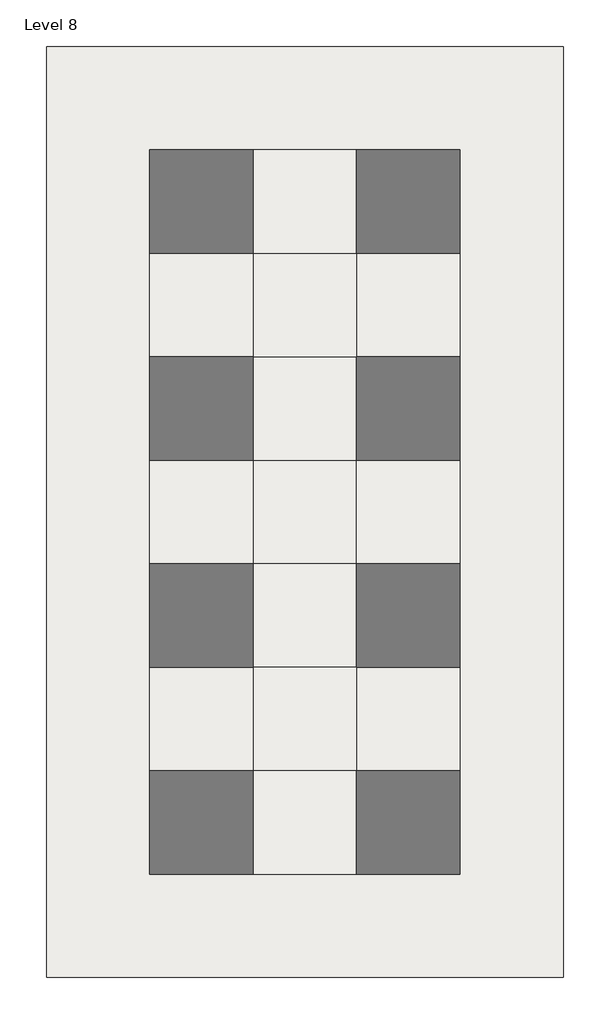
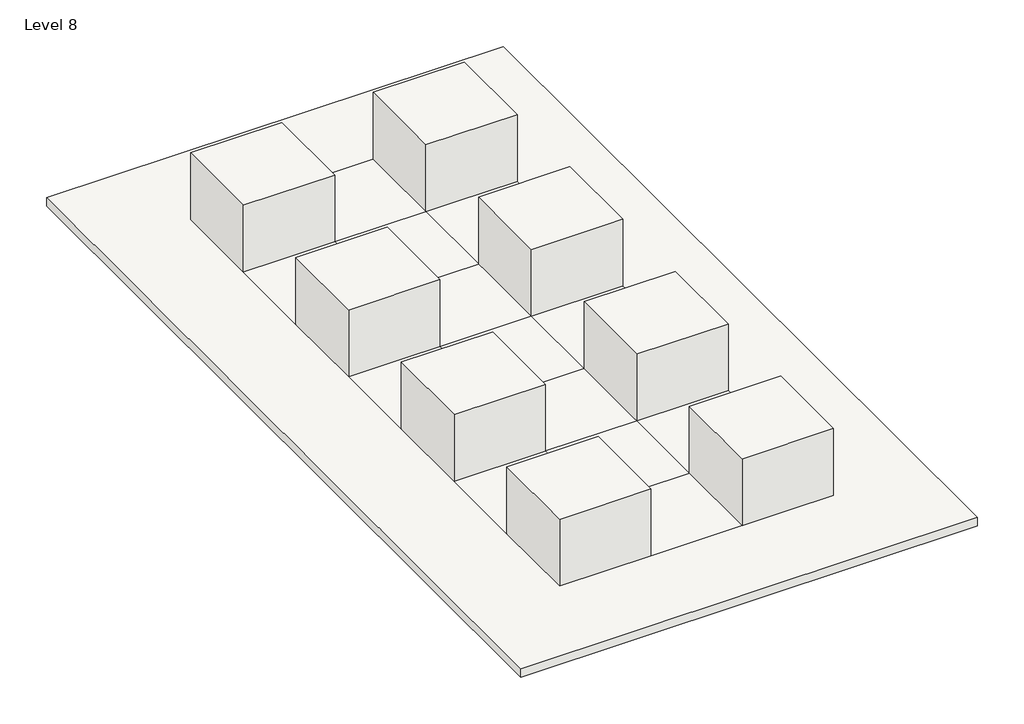
# One storey: 9 roofs.
"""IFC4 building model written with IfcOpenShell, lengths in millimetres."""

from ifc_helpers import new_model, si_unit, origin, place, context, project, spatial, faceted_brep, element, save

model = new_model("IFC4")

# Units and contexts
model_context = context("Model", 3, world=origin())
ifc_project = project(units=[si_unit("LENGTHUNIT", "METRE", prefix="MILLI")], contexts=[model_context])

# Site, building, storey
site = spatial("IfcSite", under=ifc_project)
building = spatial("IfcBuilding", under=site)
storey = spatial("IfcBuildingStorey", under=building, Name="Level 8", Elevation=32000.0)

# Roofs
placement = place(None, origin())
element("IfcRoof", 1, ObjectType="Bauder_RoofCoveringSystem_IntensiveGreenRoofSystem", at=placement, inside=storey, context=model_context, shape_type="Brep", body=[
    faceted_brep([(-674.7340554, 1676.2074539, 32000.0), (1325.2659446, 1676.2074539, 32000.0), (1325.2659446, -323.7925461, 32000.0), (-674.7340554, -323.7925461, 32000.0), (1325.2659446, 1676.2074539, 33749.8), (-674.7340554, 1676.2074539, 33749.8), (-674.7340554, -323.7925461, 33749.8), (1325.2659446, -323.7925461, 33749.8), (1325.2659446, 1676.2074539, 32200.0), (-674.7340554, 1676.2074539, 32200.0), (-674.7340554, -323.7925461, 32200.0), (1325.2659446, -323.7925461, 32200.0)], [[[0, 1, 2, 3]], [[4, 5, 6, 7]], [[5, 4, 8, 1, 0, 9]], [[6, 5, 9, 0, 3, 10]], [[7, 6, 10, 3, 2, 11]], [[4, 7, 11, 2, 1, 8]]]),
])
element("IfcRoof", 2, ObjectType="Bauder_RoofCoveringSystem_IntensiveGreenRoofSystem", at=placement, inside=storey, context=model_context, shape_type="Brep", body=[
    faceted_brep([(3325.2659446, 1676.2074539, 32000.0), (5325.2659446, 1676.2074539, 32000.0), (5325.2659446, -323.7925461, 32000.0), (3325.2659446, -323.7925461, 32000.0), (5325.2659446, 1676.2074539, 33749.8), (3325.2659446, 1676.2074539, 33749.8), (3325.2659446, -323.7925461, 33749.8), (5325.2659446, -323.7925461, 33749.8), (5325.2659446, 1676.2074539, 32200.0), (3325.2659446, 1676.2074539, 32200.0), (3325.2659446, -323.7925461, 32200.0), (5325.2659446, -323.7925461, 32200.0)], [[[0, 1, 2, 3]], [[4, 5, 6, 7]], [[5, 4, 8, 1, 0, 9]], [[6, 5, 9, 0, 3, 10]], [[7, 6, 10, 3, 2, 11]], [[4, 7, 11, 2, 1, 8]]]),
])
element("IfcRoof", 3, ObjectType="Bauder_RoofCoveringSystem_IntensiveGreenRoofSystem", at=placement, inside=storey, context=model_context, shape_type="Brep", body=[
    faceted_brep([(3325.2659446, -2323.7925461, 32000.0), (5325.2659446, -2323.7925461, 32000.0), (5325.2659446, -4323.7925461, 32000.0), (3325.2659446, -4323.7925461, 32000.0), (5325.2659446, -2323.7925461, 33749.8), (3325.2659446, -2323.7925461, 33749.8), (3325.2659446, -4323.7925461, 33749.8), (5325.2659446, -4323.7925461, 33749.8), (5325.2659446, -2323.7925461, 32200.0), (3325.2659446, -2323.7925461, 32200.0), (3325.2659446, -4323.7925461, 32200.0), (5325.2659446, -4323.7925461, 32200.0)], [[[0, 1, 2, 3]], [[4, 5, 6, 7]], [[5, 4, 8, 1, 0, 9]], [[6, 5, 9, 0, 3, 10]], [[7, 6, 10, 3, 2, 11]], [[4, 7, 11, 2, 1, 8]]]),
])
element("IfcRoof", 4, ObjectType="Bauder_RoofCoveringSystem_IntensiveGreenRoofSystem", at=placement, inside=storey, context=model_context, shape_type="Brep", body=[
    faceted_brep([(3325.2659446, -6323.7925461, 32000.0), (5325.2659446, -6323.7925461, 32000.0), (5325.2659446, -8323.7925461, 32000.0), (3325.2659446, -8323.7925461, 32000.0), (5325.2659446, -6323.7925461, 33749.8), (3325.2659446, -6323.7925461, 33749.8), (3325.2659446, -8323.7925461, 33749.8), (5325.2659446, -8323.7925461, 33749.8), (5325.2659446, -6323.7925461, 32200.0), (3325.2659446, -6323.7925461, 32200.0), (3325.2659446, -8323.7925461, 32200.0), (5325.2659446, -8323.7925461, 32200.0)], [[[0, 1, 2, 3]], [[4, 5, 6, 7]], [[5, 4, 8, 1, 0, 9]], [[6, 5, 9, 0, 3, 10]], [[7, 6, 10, 3, 2, 11]], [[4, 7, 11, 2, 1, 8]]]),
])
element("IfcRoof", 5, ObjectType="Bauder_RoofCoveringSystem_IntensiveGreenRoofSystem", at=placement, inside=storey, context=model_context, shape_type="Brep", body=[
    faceted_brep([(3325.2659446, -10323.7925461, 32000.0), (5325.2659446, -10323.7925461, 32000.0), (5325.2659446, -12323.7925461, 32000.0), (3325.2659446, -12323.7925461, 32000.0), (5325.2659446, -10323.7925461, 33749.8), (3325.2659446, -10323.7925461, 33749.8), (3325.2659446, -12323.7925461, 33749.8), (5325.2659446, -12323.7925461, 33749.8), (5325.2659446, -10323.7925461, 32200.0), (3325.2659446, -10323.7925461, 32200.0), (3325.2659446, -12323.7925461, 32200.0), (5325.2659446, -12323.7925461, 32200.0)], [[[0, 1, 2, 3]], [[4, 5, 6, 7]], [[5, 4, 8, 1, 0, 9]], [[6, 5, 9, 0, 3, 10]], [[7, 6, 10, 3, 2, 11]], [[4, 7, 11, 2, 1, 8]]]),
])
element("IfcRoof", 6, ObjectType="Bauder_RoofCoveringSystem_IntensiveGreenRoofSystem", at=placement, inside=storey, context=model_context, shape_type="Brep", body=[
    faceted_brep([(-674.7340554, -10323.7925461, 32000.0), (1325.2659446, -10323.7925461, 32000.0), (1325.2659446, -12323.7925461, 32000.0), (-674.7340554, -12323.7925461, 32000.0), (1325.2659446, -10323.7925461, 33749.8), (-674.7340554, -10323.7925461, 33749.8), (-674.7340554, -12323.7925461, 33749.8), (1325.2659446, -12323.7925461, 33749.8), (1325.2659446, -10323.7925461, 32200.0), (-674.7340554, -10323.7925461, 32200.0), (-674.7340554, -12323.7925461, 32200.0), (1325.2659446, -12323.7925461, 32200.0)], [[[0, 1, 2, 3]], [[4, 5, 6, 7]], [[5, 4, 8, 1, 0, 9]], [[6, 5, 9, 0, 3, 10]], [[7, 6, 10, 3, 2, 11]], [[4, 7, 11, 2, 1, 8]]]),
])
element("IfcRoof", 7, ObjectType="Bauder_RoofCoveringSystem_IntensiveGreenRoofSystem", at=placement, inside=storey, context=model_context, shape_type="Brep", body=[
    faceted_brep([(-674.7340554, -6323.7925461, 32000.0), (1325.2659446, -6323.7925461, 32000.0), (1325.2659446, -8323.7925461, 32000.0), (-674.7340554, -8323.7925461, 32000.0), (1325.2659446, -6323.7925461, 33749.8), (-674.7340554, -6323.7925461, 33749.8), (-674.7340554, -8323.7925461, 33749.8), (1325.2659446, -8323.7925461, 33749.8), (1325.2659446, -6323.7925461, 32200.0), (-674.7340554, -6323.7925461, 32200.0), (-674.7340554, -8323.7925461, 32200.0), (1325.2659446, -8323.7925461, 32200.0)], [[[0, 1, 2, 3]], [[4, 5, 6, 7]], [[5, 4, 8, 1, 0, 9]], [[6, 5, 9, 0, 3, 10]], [[7, 6, 10, 3, 2, 11]], [[4, 7, 11, 2, 1, 8]]]),
])
element("IfcRoof", 8, ObjectType="Bauder_RoofCoveringSystem_IntensiveGreenRoofSystem", at=placement, inside=storey, context=model_context, shape_type="Brep", body=[
    faceted_brep([(-674.7340554, -2323.7925461, 32000.0), (1325.2659446, -2323.7925461, 32000.0), (1325.2659446, -4323.7925461, 32000.0), (-674.7340554, -4323.7925461, 32000.0), (1325.2659446, -2323.7925461, 33749.8), (-674.7340554, -2323.7925461, 33749.8), (-674.7340554, -4323.7925461, 33749.8), (1325.2659446, -4323.7925461, 33749.8), (1325.2659446, -2323.7925461, 32200.0), (-674.7340554, -2323.7925461, 32200.0), (-674.7340554, -4323.7925461, 32200.0), (1325.2659446, -4323.7925461, 32200.0)], [[[0, 1, 2, 3]], [[4, 5, 6, 7]], [[5, 4, 8, 1, 0, 9]], [[6, 5, 9, 0, 3, 10]], [[7, 6, 10, 3, 2, 11]], [[4, 7, 11, 2, 1, 8]]]),
])
element("IfcRoof", 9, ObjectType="Roof_Concrete-200mm", at=placement, inside=storey, context=model_context, shape_type="Brep", body=[
    faceted_brep([(-2674.7340554, -14323.7925461, 32200.0), (-2674.7340554, -14323.7925461, 32000.0), (7325.2659446, -14323.7925461, 32000.0), (7325.2659446, -14323.7925461, 32200.0), (-2674.7340554, 3676.2074539, 32200.0), (-2674.7340554, 3676.2074539, 32000.0), (7325.2659446, 3676.2074539, 32200.0), (7325.2659446, 3676.2074539, 32000.0), (3325.2659446, 1676.2074539, 32200.0), (1325.2659446, 1676.2074539, 32200.0), (1325.2659446, -323.7925461, 32200.0), (3325.2659446, -323.7925461, 32200.0), (1325.2659446, 1676.2074539, 32000.0), (3325.2659446, 1676.2074539, 32000.0), (3325.2659446, -323.7925461, 32000.0), (1325.2659446, -323.7925461, 32000.0), (1325.2659446, -2323.7925461, 32200.0), (-674.7340554, -323.7925461, 32200.0), (-674.7340554, -2323.7925461, 32200.0), (3325.2659446, -2323.7925461, 32200.0), (5325.2659446, -2323.7925461, 32200.0), (5325.2659446, -323.7925461, 32200.0), (-674.7340554, -2323.7925461, 32000.0), (-674.7340554, -323.7925461, 32000.0), (1325.2659446, -2323.7925461, 32000.0), (3325.2659446, -2323.7925461, 32000.0), (5325.2659446, -323.7925461, 32000.0), (5325.2659446, -2323.7925461, 32000.0), (1325.2659446, -4323.7925461, 32200.0), (3325.2659446, -4323.7925461, 32200.0), (3325.2659446, -4323.7925461, 32000.0), (1325.2659446, -4323.7925461, 32000.0), (1325.2659446, -6323.7925461, 32200.0), (-674.7340554, -4323.7925461, 32200.0), (-674.7340554, -6323.7925461, 32200.0), (5325.2659446, -6323.7925461, 32200.0), (5325.2659446, -4323.7925461, 32200.0), (3325.2659446, -6323.7925461, 32200.0), (-674.7340554, -6323.7925461, 32000.0), (-674.7340554, -4323.7925461, 32000.0), (1325.2659446, -6323.7925461, 32000.0), (3325.2659446, -6323.7925461, 32000.0), (5325.2659446, -4323.7925461, 32000.0), (5325.2659446, -6323.7925461, 32000.0), (1325.2659446, -12323.7925461, 32200.0), (3325.2659446, -12323.7925461, 32200.0), (3325.2659446, -10323.7925461, 32200.0), (1325.2659446, -10323.7925461, 32200.0), (3325.2659446, -12323.7925461, 32000.0), (1325.2659446, -12323.7925461, 32000.0), (1325.2659446, -10323.7925461, 32000.0), (3325.2659446, -10323.7925461, 32000.0), (1325.2659446, -8323.7925461, 32200.0), (-674.7340554, -8323.7925461, 32200.0), (-674.7340554, -10323.7925461, 32200.0), (3325.2659446, -8323.7925461, 32200.0), (5325.2659446, -10323.7925461, 32200.0), (5325.2659446, -8323.7925461, 32200.0), (-674.7340554, -10323.7925461, 32000.0), (-674.7340554, -8323.7925461, 32000.0), (1325.2659446, -8323.7925461, 32000.0), (3325.2659446, -8323.7925461, 32000.0), (5325.2659446, -8323.7925461, 32000.0), (5325.2659446, -10323.7925461, 32000.0), (-674.7340554, 1676.2074539, 32000.0), (-674.7340554, 1676.2074539, 32200.0), (5325.2659446, 1676.2074539, 32200.0), (5325.2659446, 1676.2074539, 32000.0), (5325.2659446, -12323.7925461, 32000.0), (5325.2659446, -12323.7925461, 32200.0), (-674.7340554, -12323.7925461, 32000.0), (-674.7340554, -12323.7925461, 32200.0)], [[[0, 1, 2, 3]], [[1, 0, 4, 5]], [[6, 7, 5, 4]], [[3, 2, 7, 6]], [[8, 9, 10, 11]], [[12, 13, 14, 15]], [[16, 10, 17, 18]], [[11, 10, 16, 19]], [[20, 21, 11, 19]], [[22, 23, 15, 24]], [[15, 14, 25, 24]], [[25, 14, 26, 27]], [[19, 16, 28, 29]], [[24, 25, 30, 31]], [[32, 28, 33, 34]], [[35, 36, 29, 37]], [[38, 39, 31, 40]], [[41, 30, 42, 43]], [[44, 45, 46, 47]], [[48, 49, 50, 51]], [[47, 52, 53, 54]], [[47, 46, 55, 52]], [[56, 57, 55, 46]], [[58, 59, 60, 50]], [[51, 50, 60, 61]], [[51, 61, 62, 63]], [[52, 55, 37, 32]], [[29, 28, 32, 37]], [[61, 60, 40, 41]], [[31, 30, 41, 40]], [[9, 12, 15, 10]], [[10, 15, 23, 17]], [[17, 23, 64, 65]], [[12, 9, 65, 64]], [[66, 67, 26, 21]], [[21, 26, 14, 11]], [[11, 14, 13, 8]], [[67, 66, 8, 13]], [[20, 27, 42, 36]], [[36, 42, 30, 29]], [[29, 30, 25, 19]], [[27, 20, 19, 25]], [[16, 24, 31, 28]], [[28, 31, 39, 33]], [[33, 39, 22, 18]], [[24, 16, 18, 22]], [[32, 40, 60, 52]], [[52, 60, 59, 53]], [[53, 59, 38, 34]], [[40, 32, 34, 38]], [[35, 43, 62, 57]], [[57, 62, 61, 55]], [[55, 61, 41, 37]], [[43, 35, 37, 41]], [[56, 63, 68, 69]], [[69, 68, 48, 45]], [[45, 48, 51, 46]], [[63, 56, 46, 51]], [[47, 50, 49, 44]], [[44, 49, 70, 71]], [[71, 70, 58, 54]], [[50, 47, 54, 58]], [[4, 0, 3, 6], [9, 8, 66, 21, 20, 36, 35, 57, 56, 69, 45, 44, 71, 54, 53, 34, 33, 18, 17, 65]], [[7, 2, 1, 5], [13, 12, 64, 23, 22, 39, 38, 59, 58, 70, 49, 48, 68, 63, 62, 43, 42, 27, 26, 67]]]),
])

save(model, "model.ifc")

# Revit data of these elements
# Type "Bauder_RoofCoveringSystem_IntensiveGreenRoofSystem"
#   Keynote = "Q37"
#   Type IFC Predefined Type = "FLAT_ROOF"
#   Export Type to IFC As = "IfcRoofType"
#   Model = "Bauder Intensive Landscaping and Substrate - Intensive Green Roof System"
#   Manufacturer = "Bauder Ltd"
#   Type Comments = "Intensive Green Roof System"
#   URL = "http://www.bauder.co.uk/"
#   Description = "Bauder Intensive GreenRoof system incorporating Intensive Landscaping with Intensive Substrate, Filter Fleece, Mineral Drain, DSE60 Polyethylene Drainage and Protection Layer, FSM 1100 protection mat and PE Foil Polyethylene Separation-Slip Layer"
#   Assembly Code = "B3010"
#   NBSDescription = "Intensive green roof system"
#   NBSReference = "45-40-47/110"
#   BIMObjectName = "Bauder_RoofCoveringSystem_IntensiveGreenRoofSystem"
#   AccessibilityPerformance = "n/a"
#   CodePerformance = "n/a"
#   Color = "n/a"
#   Constituents = "n/a"
#   DurationUnit = "Year"
#   ExpectedLife = "n/a"
#   Features = "This BIM Object must be supported by a project specific specification from Bauder, incorporating system build-up, detail design and performance calculations if a full Bauder system guarantee is required. Please contact your local Bauder Representative or technical@bauder.co.uk"
#   Finish = "n/a"
#   Grade = "n/a"
#   Material = "n/a"
#   ModelReference = "Bauder Intensive Landscaping and Substrate - Intensive Green Roof System"
#   Name = "RoofCoveringSystem_Bauder_IntensiveGreenRoofSystem"
#   ReplacementCost = "n/a"
#   Shape = "n/a"
#   Size = "n/a"
#   SustainabilityPerformance = "Bauder Germany ISO14001: Certificate No.: 70499/03-15 e, Bauder UK ISO14001:Certificate No. 19ACM6595R, EN1271, BREEAM Credits Available"
#   WarrantyDescription = "Guarantee options could include ‘Product’, ‘Product and Workmanship’ and ‘Product, Workmanship and Design’ Guarantees. All guarantees available for this system are subject to the works being carried out in accordance with the Bauder specification and being installed by a Bauder Approved installer. For full details and further information regarding guarantees and alternative systems please contact your local Bauder Representative or technical@bauder.co.uk"
#   WarrantyDurationLabor = "n/a"
#   WarrantyDurationParts = "n/a\r\nn/a"
#   WarrantyDurationUnit = "Year"
#   WarrantyGuarantorLabor = "n/a"
#   WarrantyGuarantorParts = "technical@bauder.co.uk"
#   Certification = "n/a"
#   EdgeRestraints = "Perforated edge trim where required, refer to Bauder Project Specific Specification"
#   MoistureControlDrainageAncillaries = "n/a"
#   MoistureControlDrainageLayer = "Bauder DSE60 60 mm Polyethylene Drainage and Protection Layer with Bauder Mineral Drain Single size stone aggregate infill"
#   MoistureControlFilterMembrane = "Bauder Filter Fleece 1 mm Polypropylene Filter Fleece"
#   MoistureControlMoistureRetentionMat = "n/a"
#   PlantingSystemsAntierosionMat = "Jute Net where exposed, refer to Bauder Project Specific Specification"
#   PlantingSystemsPlantingMedium = "Bauder Intensive Substrate Recycled crushed brick, expanded clay shale and composted pine bark"
#   PlantingSystemsVegetation = "Bauder Intensive Landscaping"
#   PlantingSystemsVegetationBarrier = "20-40 mm Rounded-Washed Stones, refer to Bauder Project Specific Specification"
#   ProjectSpecificationAndDesign = "This BIM Object must be supported by a project specific specification from Bauder, incorporating system build-up, detail design and performance calculations if a full Bauder system warranty is required. Please contact your local Bauder Representative or technical@bauder.co.uk"
#   ProtectionProtectionLayer = "BauderGREEN FSM 1100 Protection Mat"
#   ProtectionRootBarrier = "As per project specific Bauder Specification"
#   ProtectionSeparationLayer = "2 layers of Bauder PE Foil 0.2 mm Polyethylene Separation-Slip Layer"
#   SystemManufacturer = "Bauder Ltd"
#   WarrantyConsiderations = "All guarantees available for this system are subject to the works being carried out in accordance with the Bauder specification and being installed by a Bauder Approved installer. For full details and further information regarding guarantees and alternative systems please contact your local Bauder Representative or technical@bauder.co.uk"
#   Update = "1900-12-31T23:59:59"
#   Documentation = "https://www.bauder.co.uk/technical-centre/technical-literature/system-brochures"
#   DocumentReference = "http://www.bauder.co.uk/"
#   IfcExportAs = "IfcRoofType"
#   IfcExportType = "FLAT_ROOF"
#   MethodOfMesurement = "n/a"
#   Process = "Replacement at service life intervals"
#   FireRating = "n/a"
#   _Author = "AM"
#   _AuthorizedBy = "bimstore"
#   _CreatedBy = "technical@bauder.co.uk"
#   _DistributedBy = "www.bimstore.co"
#   AssetType = "Fixed"
#   ClassificationName = "Uniclass2015"
#   ClassificationValue = "Ss_45_40_47_40"
#   CreatedBy = "technical@bauder.co.uk"
#   CreatedOn = "2023-02-10 T00:00:00"
#   DocumentationCertificates = "n/a"
#   DocumentationInstallationGuide = "https://www.bauder.co.uk/technical-centre"
#   DocumentationLiterature = "https://www.bauder.co.uk/technical-centre"
#   DocumentationMaintenance = "https://www.bauder.co.uk/technical-centre/maintenance-advice"
#   DocumentationTechnical = "https://www.bauder.co.uk/green-roofs/intensive-green-roofs"
#   ManufacturerName = "Bauder Ltd"
#   ModelNumber = "0910_INT-InS-FF-D6-F11-PE"
#   ProductionYear = "2023"
#   ReferencedStandard = "n/a"
#   SpareParts = "n/a"
#   TypeName = "Intensive Green Roof System"
#   NBSNote = "n/a"
#   NBSObjectName = "Bauder - Intensive green roof system"
#   NBSOfficeMasterTag = "n/a"
#   Ballast = "n/a"
#   CarrierMembraneFixing = "n/a"
#   CarrierMembraneType = "n/a"
#   FillToPerimeterUpstands = "n/a"
#   FilterLayer = "n/a"
#   InsulationFixing = "n/a"
#   InsulationType = "n/a"
#   LiquidAppliedWaterproofCoatingReinforcement = "n/a"
#   LiquidAppliedWaterproofCoatingSurfaceTreatment = "n/a"
#   LiquidAppliedWaterproofCoatingType = "n/a"
#   PreparationExistingSubstrates = "n/a"
#   PreparationHorizontalWork = "n/a"
#   PreparationSkirtingsAndVerticalWork = "n/a"
#   ProtectionLayer = "n/a"
#   SystemAccessories = "n/a"
#   WaterproofCoveringFirstLayerAttachment = "n/a"
#   WaterproofCoveringFirstLayerType = "n/a"
#   WaterproofCoveringIntermediateLayerAttachment = "n/a"
#   WaterproofCoveringIntermediateLayerType = "n/a"
#   WaterproofCoveringTopLayerAttachment = "n/a"
#   InsulationAttachment = "n/a"
#   IsolatingLayer = "n/a"
#   CarrierMembraneAttachment = "n/a"
#   LiquidAppliedWaterproofCoatingWearingCourse = "n/a"
#   VapourControlLayer = "n/a"
#   VapourControlLayerAttachment_Bauder = "n/a"
#   WaterproofCoveringJoints = "n/a"
#   WaterproofCoveringType = "n/a"
#   SeparatingLayer = "n/a"
#   WaterproofCoveringAccessories = "Yes"
#   WaterproofCoveringAttachment = "n/a"
#   UpperProtectionLayer = "n/a"
#   LowerProtectionLayer = "n/a"
#   WaterproofCoveringTopLayerType = "n/a"
#   DetailWorkAncillaryItems = "Detail as per project specific Bauder Specification"
#   DetailWorkCoverStrips = "Detail as per project specific Bauder Specification"
#   DetailWorkFlashings = "Detail as per project specific Bauder Specification"
#   DetailWorkSkirtingsAndUpstands = "Detail as per project specific Bauder Specification"
#   DetailWorkWeltedDrips = "Detail as per project specific Bauder Specification"
#   OverlayFixing = "n/a"
#   OverlayType = "n/a"
#   SurfaceProtection = "n/a"
#   VapourControlLayerAttachment = "n/a"
#   VapourControlLayerType = "n/a"
#   Cost = 0
#   NominalHeight = 0 mm
#   NominalLength = 0 mm
#   TotalArea = 0 m²
#   NominalDepth = 0 mm
#   IsExternal = yes
#   _BimSpecGuid = 0
#   _BSBibleVersion = 16
#   _CurrentRevision = 4
#   Layers, outside or top first: 700 mm "Bauder_Landscaping_Intensive" (function 5); 800 mm "Bauder_IntensiveSubstrate_BauderGREEN-SUB-IM-UK" (function 2); 1 mm "Bauder_FilterFleece_BauderGREEN-FV-125-100" (function 2); 40 mm "Bauder_DrainageBoard_BauderGREEN-DSE-40" (function 3); 8 mm "Bauder_ProtectionMat_BauderGREEN-FSM1100" (function 3); 200 mm "Concrete" (function 1); 0.8 mm "Bauder_SeparationAndSlipLayer_BauderGREEN-PE-02" (function 3)
# Type "Roof_Concrete-200mm"
#   Layers, outside or top first: 200 mm "Concrete" (function 1)
# Elements 1, 2, 3, 4, 5, 6, 7, 8 (IfcRoof, "Bauder_RoofCoveringSystem_IntensiveGreenRoofSystem")
#   built-in parameter 1001705 = 110.728 (stored number, unit not read)
#   built-in parameter 1001710 = 33615
#   Phase Created = New Construction
#   Materials on its faces: "Bauder_SeparationAndSlipLayer_BauderGREEN-PE-02", "Bauder_Landscaping_Intensive"
# Element 9 (IfcRoof, "Roof_Concrete-200mm")
#   built-in parameter 1001710 = 33615
#   Phase Created = New Construction
#   Materials on its faces: "Concrete"
# Materials
#   "Bauder_Landscaping_Intensive": class "Unassigned", colour RGB 62 68 37, transparency 0, Mtrl_Author = "AM", Mtrl_AuthorizedBy = "bimstore", Mtrl_DistributedBy = "www.bimstore.co", Mtrl_AccessibilityPerformance = "n/a", Mtrl_AssetIdentifier = "Please record on commissioning", Mtrl_AssetType = "Fixed", Mtrl_BarCode = "Please record on commissioning", Mtrl_ClassificationName = "Uniclass2015", Mtrl_ClassificationValue = "n/a", Mtrl_CodePerformance = "n/a", Mtrl_Color = "n/a", Mtrl_Constituents = "n/a", Mtrl_CreatedBy = "technical@bauder.co.uk", Mtrl_CreatedOn = "2023-02-10 T00:00:00", Mtrl_DocumentationCertificates = "https://www.bimstore.co/products/intensive-green-roof-system/document/product-certificates", Mtrl_DocumentationInstallationGuide = "https://www.bimstore.co/products/intensive-green-roof-system/document/installation-guide", Mtrl_DocumentationLiterature = "https://www.bimstore.co/products/intensive-green-roof-system/document/product-literature", Mtrl_DocumentationMaintenance = "https://www.bimstore.co/products/intensive-green-roof-system/document/maintenance-information", Mtrl_DocumentationTechnical = "https://www.bimstore.co/products/intensive-green-roof-system/document/technical-data-sheet", Mtrl_DurationUnit = "Year", Mtrl_Features = "n/a", Mtrl_Finish = "n/a", Mtrl_Grade = "n/a", Mtrl_InstallationDate = "Please record on commissioning", Mtrl_ManufacturerName = "Bauder Ltd", Mtrl_Material = "n/a", Mtrl_ModelNumber = "Intensive", Mtrl_ModelReference = "Landscaping", Mtrl_ProductionYear = "2023", Mtrl_ReferencedStandard = "n/a", Mtrl_Shape = "n/a", Mtrl_Size = "n/a", Mtrl_SpareParts = "n/a", Mtrl_TypeName = "Intensive", Mtrl_WarrantyDescription = "n/a", Mtrl_WarrantyDurationUnit = "Year", Mtrl_WarrantyGuarantorLabor = "n/a", Mtrl_WarrantyGuarantorParts = "technical@bauder.co.uk", Mtrl_WarrantyStartDate = "Please record on commissioning", Mtrl_IfcExportAs = "IfcRoofType", Mtrl_IfcExportType = "FLAT_ROOF", Mtrl_BIMObjectName = "Bauder_Landscaping_Intensive", Mtrl_NBSDescription = "n/a", Mtrl_NBSNote = "n/a", Mtrl_NBSObjectName = "n/a", Mtrl_NBSOfficeMasterTag = "n/a", Mtrl_NBSReference = "Q37", Mtrl_Ballast = "n/a", Mtrl_CarrierMembraneAttachment = "n/a", Mtrl_CarrierMembraneFixing = "n/a", Mtrl_CarrierMembraneType = "n/a", Mtrl_Certification = "Comply with GRO Green Roof Code of Practice and FLL Standards", Mtrl_DetailWorkAncillaryItems = "Detail as per project specific Bauder Specification", Mtrl_DetailWorkCoverStrips = "Detail as per project specific Bauder Specification", Mtrl_DetailWorkFlashings = "Detail as per project specific Bauder Specification", Mtrl_DetailWorkSkirtingsAndUpstands = "Detail as per project specific Bauder Specification", Mtrl_DetailWorkWeltedDrips = "Detail as per project specific Bauder Specification", Mtrl_EdgeRestraints = "Detail as per project specific Bauder Specification", Mtrl_FillToPerimeterUpstands = "n/a", Mtrl_FilterLayer = "n/a", Mtrl_InsulationAttachment = "As per project specific Bauder Specification", Mtrl_InsulationFixing = "As per project specific Bauder Specification", Mtrl_InsulationType = "As per project specific Bauder Specification", Mtrl_IsolatingLayer = "n/a", Mtrl_LiquidAppliedWaterproofCoatingReinforcement = "n/a", Mtrl_LiquidAppliedWaterproofCoatingSurfaceTreatment = "As per project specific Bauder Specification", Mtrl_LiquidAppliedWaterproofCoatingType = "As per project specific Bauder Specification", Mtrl_LiquidAppliedWaterproofCoatingWearingCourse = "As per project specific Bauder Specification", Mtrl_LowerProtectionLayer = "n/a", Mtrl_MoistureControlDrainageAncillaries = "n/a", Mtrl_MoistureControlDrainageLayer = "n/a", Mtrl_MoistureControlFilterMembrane = "n/a", Mtrl_MoistureControlMoistureRetentionMat = "n/a", Mtrl_OverlayFixing = "n/a", Mtrl_OverlayType = "n/a", Mtrl_PlantingSystemsAntierosionMat = "n/a", Mtrl_PlantingSystemsPlantingMedium = "As per project specific Bauder Specification", Mtrl_PlantingSystemsVegetation = "As per project specific Bauder Specification", Mtrl_PlantingSystemsVegetationBarrier = "As per project specific Bauder Specification", Mtrl_PreparationExistingSubstrates = "n/a", Mtrl_PreparationHorizontalWork = "n/a", Mtrl_PreparationSkirtingsAndVerticalWork = "n/a", Mtrl_ProjectSpecificationAndDesign = "This BIM Object must be supported by a project specific specification from Bauder, incorporating system build-up, detail design and performance calculations if a full Bauder system warranty is required. Please contact your local Bauder Representative or technical@bauder.co.uk", Mtrl_ProtectionLayer = "n/a", Mtrl_ProtectionProtectionLayer = "n/a", Mtrl_ProtectionRootBarrier = "As per project specific Bauder Specification", Mtrl_ProtectionSeparationLayer = "n/a", Mtrl_SeparatingLayer = "n/a", Mtrl_SurfaceProtection = "n/a", Mtrl_SystemAccessories = "n/a", Mtrl_SystemManufacturer = "Bauder Ltd", Mtrl_Update = "1900-12-31 T23:59:59", Mtrl_UpperProtectionLayer = "n/a", Mtrl_VapourControlLayerAttachment = "As per project specific Bauder Specification", Mtrl_VapourControlLayerAttachment_Bauder = "As per project specific Bauder Specification", Mtrl_VapourControlLayerType = "As per project specific Bauder Specification", Mtrl_WarrantyConsiderations = "All guarantees available for this system are subject to the works being carried out in accordance with the Bauder specification and being installed by a Bauder Approved installer. For full details and further information regarding guarantees and alternative systems please contact your local Bauder Representative or technical@bauder.co.uk", Mtrl_WaterproofCoveringAccessories = "As per project specific Bauder Specification", Mtrl_WaterproofCoveringAttachment = "As per project specific Bauder Specification", Mtrl_WaterproofCoveringFirstLayerAttachment = "As per project specific Bauder Specification", Mtrl_WaterproofCoveringFirstLayerType = "As per project specific Bauder Specification", Mtrl_WaterproofCoveringIntermediateLayerAttachment = "As per project specific Bauder Specification", Mtrl_WaterproofCoveringIntermediateLayerType = "As per project specific Bauder Specification", Mtrl_WaterproofCoveringJoints = "As per project specific Bauder Specification", Mtrl_WaterproofCoveringTopLayerAttachment = "As per project specific Bauder Specification", Mtrl_WaterproofCoveringTopLayerType = "As per project specific Bauder Specification", Mtrl_WaterproofCoveringType = "As per project specific Bauder Specification", Cost = 0, Mtrl_ReplacementCost = 0, Mtrl_NominalDepth = 0 mm, Mtrl_NominalHeight = 0 mm, Mtrl_NominalLength = 0 mm, Mtrl_BimSpecGuid = 0, Mtrl_BSBibleVersion = 17, Mtrl_CurrentRevision = 2, Mtrl_ExpectedLife = 0, Mtrl_SerialNumber = 0, Mtrl_WarrantyDurationLabor = 0, Mtrl_WarrantyDurationParts = 0
#   "Bauder_IntensiveSubstrate_BauderGREEN-SUB-IM-UK": class "Unassigned", colour RGB 255 255 255, transparency 0, Mtrl_Author = "AM", Mtrl_AuthorizedBy = "bimstore", Mtrl_DistributedBy = "www.bimstore.co", Mtrl_AccessibilityPerformance = "n/a", Mtrl_AssetIdentifier = "Please record on commissioning", Mtrl_AssetType = "Fixed", Mtrl_BarCode = "Please record on commissioning", Mtrl_ClassificationName = "Uniclass2015", Mtrl_ClassificationValue = "n/a", Mtrl_CodePerformance = "n/a", Mtrl_Color = "n/a", Mtrl_Constituents = "n/a", Mtrl_CreatedBy = "technical@bauder.co.uk", Mtrl_CreatedOn = "2023-02-10 T00:00:00", Mtrl_DocumentationCertificates = "https://www.bimstore.co/products/intensive-green-roof-system/document/product-certificates", Mtrl_DocumentationInstallationGuide = "https://www.bimstore.co/products/intensive-green-roof-system/document/installation-guide", Mtrl_DocumentationLiterature = "https://www.bimstore.co/products/intensive-green-roof-system/document/product-literature", Mtrl_DocumentationMaintenance = "https://www.bimstore.co/products/intensive-green-roof-system/document/maintenance-information", Mtrl_DocumentationTechnical = "https://www.bimstore.co/products/intensive-green-roof-system/document/technical-data-sheet", Mtrl_DurationUnit = "Year", Mtrl_Features = "n/a", Mtrl_Finish = "n/a", Mtrl_Grade = "n/a", Mtrl_InstallationDate = "Please record on commissioning", Mtrl_ManufacturerName = "Bauder Ltd", Mtrl_Material = "Expanded Clay Aggregate", Mtrl_ModelNumber = "BauderGREEN-SUB-IM-UK", Mtrl_ModelReference = "Intensive Substrate", Mtrl_ProductionYear = "2023", Mtrl_ReferencedStandard = "n/a", Mtrl_Shape = "n/a", Mtrl_Size = "n/a", Mtrl_SpareParts = "n/a", Mtrl_TypeName = "BauderGREEN-SUB-IM-UK", Mtrl_WarrantyDescription = "As part of Bauder system guarantee, per specification", Mtrl_WarrantyDurationUnit = "Year", Mtrl_WarrantyGuarantorLabor = "n/a", Mtrl_WarrantyGuarantorParts = "technical@bauder.co.uk", Mtrl_WarrantyStartDate = "Please record on commissioning", Mtrl_IfcExportAs = "IfcRoofType", Mtrl_IfcExportType = "FLAT_ROOF", Mtrl_BIMObjectName = "Bauder_IntensiveSubstrate_BauderGREEN-SUB-IM-UK", Mtrl_NBSDescription = "n/a", Mtrl_NBSNote = "n/a", Mtrl_NBSObjectName = "n/a", Mtrl_NBSOfficeMasterTag = "n/a", Mtrl_NBSReference = "Q37", Mtrl_Ballast = "n/a", Mtrl_CarrierMembraneAttachment = "n/a", Mtrl_CarrierMembraneFixing = "n/a", Mtrl_CarrierMembraneType = "n/a", Mtrl_Certification = "Comply with GRO Green Roof Code of Practice and FLL Standards", Mtrl_DetailWorkAncillaryItems = "Detail as per project specific Bauder Specification", Mtrl_DetailWorkCoverStrips = "Detail as per project specific Bauder Specification", Mtrl_DetailWorkFlashings = "Detail as per project specific Bauder Specification", Mtrl_DetailWorkSkirtingsAndUpstands = "Detail as per project specific Bauder Specification", Mtrl_DetailWorkWeltedDrips = "Detail as per project specific Bauder Specification", Mtrl_EdgeRestraints = "Detail as per project specific Bauder Specification", Mtrl_FillToPerimeterUpstands = "n/a", Mtrl_FilterLayer = "n/a", Mtrl_InsulationAttachment = "As per project specific Bauder Specification", Mtrl_InsulationFixing = "As per project specific Bauder Specification", Mtrl_InsulationType = "As per project specific Bauder Specification", Mtrl_IsolatingLayer = "n/a", Mtrl_LiquidAppliedWaterproofCoatingReinforcement = "As per project specific Bauder Specification", Mtrl_LiquidAppliedWaterproofCoatingSurfaceTreatment = "As per project specific Bauder Specification", Mtrl_LiquidAppliedWaterproofCoatingType = "As per project specific Bauder Specification", Mtrl_LiquidAppliedWaterproofCoatingWearingCourse = "As per project specific Bauder Specification", Mtrl_LowerProtectionLayer = "n/a", Mtrl_MoistureControlDrainageAncillaries = "n/a", Mtrl_MoistureControlDrainageLayer = "n/a", Mtrl_MoistureControlFilterMembrane = "n/a", Mtrl_MoistureControlMoistureRetentionMat = "n/a", Mtrl_OverlayFixing = "n/a", Mtrl_OverlayType = "n/a", Mtrl_PlantingSystemsAntierosionMat = "n/a", Mtrl_PlantingSystemsPlantingMedium = "As per project specific Bauder Specification", Mtrl_PlantingSystemsVegetation = "As per project specific Bauder Specification", Mtrl_PlantingSystemsVegetationBarrier = "As per project specific Bauder Specification", Mtrl_PreparationExistingSubstrates = "n/a", Mtrl_PreparationHorizontalWork = "n/a", Mtrl_PreparationSkirtingsAndVerticalWork = "n/a", Mtrl_ProjectSpecificationAndDesign = "This BIM Object must be supported by a project specific specification from Bauder, incorporating system build-up, detail design and performance calculations if a full Bauder system warranty is required. Please contact your local Bauder Representative or technical@bauder.co.uk", Mtrl_ProtectionLayer = "n/a", Mtrl_ProtectionProtectionLayer = "n/a", Mtrl_ProtectionRootBarrier = "As per project specific Bauder Specification", Mtrl_ProtectionSeparationLayer = "n/a", Mtrl_SeparatingLayer = "n/a", Mtrl_SurfaceProtection = "n/a", Mtrl_SystemAccessories = "n/a", Mtrl_SystemManufacturer = "Bauder Ltd", Mtrl_Update = "1900-12-31 T23:59:59", Mtrl_UpperProtectionLayer = "n/a", Mtrl_VapourControlLayerAttachment = "As per project specific Bauder Specification", Mtrl_VapourControlLayerAttachment_Bauder = "As per project specific Bauder Specification", Mtrl_VapourControlLayerType = "As per project specific Bauder Specification", Mtrl_WarrantyConsiderations = "All guarantees available for this system are subject to the works being carried out in accordance with the Bauder specification and being installed by a Bauder Approved installer. For full details and further information regarding guarantees and alternative systems please contact your local Bauder Representative or technical@bauder.co.uk", Mtrl_WaterproofCoveringAccessories = "As per project specific Bauder Specification", Mtrl_WaterproofCoveringAttachment = "As per project specific Bauder Specification", Mtrl_WaterproofCoveringFirstLayerAttachment = "As per project specific Bauder Specification", Mtrl_WaterproofCoveringFirstLayerType = "As per project specific Bauder Specification", Mtrl_WaterproofCoveringIntermediateLayerAttachment = "As per project specific Bauder Specification", Mtrl_WaterproofCoveringIntermediateLayerType = "As per project specific Bauder Specification", Mtrl_WaterproofCoveringJoints = "As per project specific Bauder Specification", Mtrl_WaterproofCoveringTopLayerAttachment = "As per project specific Bauder Specification", Mtrl_WaterproofCoveringTopLayerType = "As per project specific Bauder Specification", Mtrl_WaterproofCoveringType = "As per project specific Bauder Specification", Cost = 0, Mtrl_ReplacementCost = 0, Mtrl_NominalDepth = 200 mm, Mtrl_NominalHeight = 0 mm, Mtrl_NominalLength = 0 mm, Mtrl_BimSpecGuid = 0, Mtrl_BSBibleVersion = 17, Mtrl_CurrentRevision = 2, Mtrl_ExpectedLife = 0, Mtrl_SerialNumber = 0, Mtrl_WarrantyDurationLabor = 0, Mtrl_WarrantyDurationParts = 0
#   "Bauder_FilterFleece_BauderGREEN-FV-125-100": class "Unassigned", colour RGB 255 255 255, transparency 0, Mtrl_Author = "AM", Mtrl_AuthorizedBy = "bimstore", Mtrl_DistributedBy = "www.bimstore.co", Mtrl_AccessibilityPerformance = "n/a", Mtrl_AssetIdentifier = "Please record on commissioning", Mtrl_AssetType = "Fixed", Mtrl_BarCode = "Please record on commissioning", Mtrl_ClassificationName = "Uniclass2015", Mtrl_ClassificationValue = "n/a", Mtrl_CodePerformance = "n/a", Mtrl_Color = "n/a", Mtrl_Constituents = "n/a", Mtrl_CreatedBy = "technical@bauder.co.uk", Mtrl_CreatedOn = "2023-02-10 T00:00:00", Mtrl_DocumentationCertificates = "https://www.bimstore.co/products/extensive-green-roof-system-wildflower-blanket/document/product-certificates", Mtrl_DocumentationInstallationGuide = "https://www.bimstore.co/products/extensive-green-roof-system-wildflower-blanket/document/installation-guide", Mtrl_DocumentationLiterature = "https://www.bimstore.co/products/intensive-green-roof-system/document/product-literature", Mtrl_DocumentationMaintenance = "https://www.bimstore.co/products/extensive-green-roof-system-wildflower-blanket/document/maintenance-information", Mtrl_DocumentationTechnical = "https://www.bimstore.co/products/extensive-green-roof-system-wildflower-blanket/document/technical-data-sheet", Mtrl_DurationUnit = "Year", Mtrl_Features = "n/a", Mtrl_Finish = "n/a", Mtrl_Grade = "n/a", Mtrl_InstallationDate = "Please record on commissioning", Mtrl_ManufacturerName = "Bauder Ltd", Mtrl_Material = "Polypropylene Fleece", Mtrl_ModelNumber = "BauderGREEN-FV-125-100", Mtrl_ModelReference = "Filter Fleece", Mtrl_ProductionYear = "2023", Mtrl_ReferencedStandard = "n/a", Mtrl_Shape = "n/a", Mtrl_Size = "n/a", Mtrl_SpareParts = "n/a", Mtrl_TypeName = "BauderGREEN-FV-125-100", Mtrl_WarrantyDescription = "As part of Bauder system guarantee, per specification", Mtrl_WarrantyDurationUnit = "Year", Mtrl_WarrantyGuarantorLabor = "technical@bauder.co.uk", Mtrl_WarrantyGuarantorParts = "technical@bauder.co.uk", Mtrl_WarrantyStartDate = "Please record on commissioning", Mtrl_IfcExportAs = "IfcRoofType", Mtrl_IfcExportType = "FLAT_ROOF", Mtrl_BIMObjectName = "Bauder_FilterFleece_BauderGREEN-FV-125-100", Mtrl_NBSDescription = "n/a", Mtrl_NBSNote = "n/a", Mtrl_NBSObjectName = "n/a", Mtrl_NBSOfficeMasterTag = "n/a", Mtrl_NBSReference = "Q37", Mtrl_Ballast = "n/a", Mtrl_CarrierMembraneAttachment = "n/a", Mtrl_CarrierMembraneFixing = "n/a", Mtrl_CarrierMembraneType = "n/a", Mtrl_Certification = "Comply with GRO Green Roof Code of Practice and FLL Standards", Mtrl_DetailWorkAncillaryItems = "Detail as per project specific Bauder Specification", Mtrl_DetailWorkCoverStrips = "Detail as per project specific Bauder Specification", Mtrl_DetailWorkFlashings = "Detail as per project specific Bauder Specification", Mtrl_DetailWorkSkirtingsAndUpstands = "Detail as per project specific Bauder Specification", Mtrl_DetailWorkWeltedDrips = "Detail as per project specific Bauder Specification", Mtrl_EdgeRestraints = "Detail as per project specific Bauder Specification", Mtrl_FillToPerimeterUpstands = "n/a", Mtrl_FilterLayer = "n/a", Mtrl_InsulationAttachment = "As per project specific Bauder Specification", Mtrl_InsulationFixing = "As per project specific Bauder Specification", Mtrl_InsulationType = "As per project specific Bauder Specification", Mtrl_IsolatingLayer = "n/a", Mtrl_LiquidAppliedWaterproofCoatingReinforcement = "As per project specific Bauder Specification", Mtrl_LiquidAppliedWaterproofCoatingSurfaceTreatment = "As per project specific Bauder Specification", Mtrl_LiquidAppliedWaterproofCoatingType = "As per project specific Bauder Specification", Mtrl_LiquidAppliedWaterproofCoatingWearingCourse = "As per project specific Bauder Specification", Mtrl_LowerProtectionLayer = "n/a", Mtrl_MoistureControlDrainageAncillaries = "n/a", Mtrl_MoistureControlDrainageLayer = "n/a", Mtrl_MoistureControlFilterMembrane = "n/a", Mtrl_MoistureControlMoistureRetentionMat = "n/a", Mtrl_OverlayFixing = "n/a", Mtrl_OverlayType = "n/a", Mtrl_PlantingSystemsAntierosionMat = "n/a", Mtrl_PlantingSystemsPlantingMedium = "As per project specific Bauder Specification", Mtrl_PlantingSystemsVegetation = "As per project specific Bauder Specification", Mtrl_PlantingSystemsVegetationBarrier = "As per project specific Bauder Specification", Mtrl_PreparationExistingSubstrates = "n/a", Mtrl_PreparationHorizontalWork = "n/a", Mtrl_PreparationSkirtingsAndVerticalWork = "n/a", Mtrl_ProjectSpecificationAndDesign = "This BIM Object must be supported by a project specific specification from Bauder, incorporating system build-up, detail design and performance calculations if a full Bauder system warranty is required. Please contact your local Bauder Representative or technical@bauder.co.uk", Mtrl_ProtectionLayer = "n/a", Mtrl_ProtectionProtectionLayer = "n/a", Mtrl_ProtectionRootBarrier = "As per project specific Bauder Specification", Mtrl_ProtectionSeparationLayer = "n/a", Mtrl_SeparatingLayer = "n/a", Mtrl_SurfaceProtection = "n/a", Mtrl_SystemAccessories = "n/a", Mtrl_SystemManufacturer = "Bauder Ltd", Mtrl_Update = "1900-12-31 T23:59:59", Mtrl_UpperProtectionLayer = "n/a", Mtrl_VapourControlLayerAttachment = "As per project specific Bauder Specification", Mtrl_VapourControlLayerAttachment_Bauder = "As per project specific Bauder Specification", Mtrl_VapourControlLayerType = "As per project specific Bauder Specification", Mtrl_WarrantyConsiderations = "All guarantees available for this system are subject to the works being carried out in accordance with the Bauder specification and being installed by a Bauder Approved installer. For full details and further information regarding guarantees and alternative systems please contact your local Bauder Representative or technical@bauder.co.uk", Mtrl_WaterproofCoveringAccessories = "As per project specific Bauder Specification", Mtrl_WaterproofCoveringAttachment = "As per project specific Bauder Specification", Mtrl_WaterproofCoveringFirstLayerAttachment = "As per project specific Bauder Specification", Mtrl_WaterproofCoveringFirstLayerType = "As per project specific Bauder Specification", Mtrl_WaterproofCoveringIntermediateLayerAttachment = "As per project specific Bauder Specification", Mtrl_WaterproofCoveringIntermediateLayerType = "As per project specific Bauder Specification", Mtrl_WaterproofCoveringJoints = "As per project specific Bauder Specification", Mtrl_WaterproofCoveringTopLayerAttachment = "As per project specific Bauder Specification", Mtrl_WaterproofCoveringTopLayerType = "As per project specific Bauder Specification", Mtrl_WaterproofCoveringType = "As per project specific Bauder Specification", Cost = 0, Mtrl_ReplacementCost = 0, Mtrl_NominalDepth = 1 mm, Mtrl_NominalHeight = 0 mm, Mtrl_NominalLength = 0 mm, Mtrl_BimSpecGuid = 0, Mtrl_BSBibleVersion = 17, Mtrl_CurrentRevision = 2, Mtrl_ExpectedLife = 0, Mtrl_SerialNumber = 0, Mtrl_WarrantyDurationLabor = 0, Mtrl_WarrantyDurationParts = 0
#   "Bauder_DrainageBoard_BauderGREEN-DSE-40": class "Unassigned", colour RGB 255 255 255, transparency 0, Mtrl_Author = "AM", Mtrl_AuthorizedBy = "bimstore", Mtrl_DistributedBy = "www.bimstore.co", Mtrl_AccessibilityPerformance = "n/a", Mtrl_AssetIdentifier = "Please record on commissioning", Mtrl_AssetType = "Fixed", Mtrl_BarCode = "Please record on commissioning", Mtrl_ClassificationName = "Uniclass2015", Mtrl_ClassificationValue = "Pr_65_67_78_72", Mtrl_CodePerformance = "n/a", Mtrl_Color = "n/a", Mtrl_Constituents = "n/a", Mtrl_CreatedBy = "technical@bauder.co.uk", Mtrl_CreatedOn = "2023-02-10 T00:00:00", Mtrl_DocumentationCertificates = "https://www.bimstore.co/products/extensive-green-roof-system-wildflower-blanket/document/product-certificates", Mtrl_DocumentationInstallationGuide = "https://www.bimstore.co/products/extensive-green-roof-system-wildflower-blanket/document/installation-guide", Mtrl_DocumentationLiterature = "https://www.bimstore.co/products/extensive-green-roof-system-wildflower-blanket/document/product-literature", Mtrl_DocumentationMaintenance = "https://www.bimstore.co/products/extensive-green-roof-system-wildflower-blanket/document/maintenance-information", Mtrl_DocumentationTechnical = "https://www.bimstore.co/products/extensive-green-roof-system-wildflower-blanket/document/technical-data-sheet", Mtrl_DurationUnit = "Year", Mtrl_Features = "n/a", Mtrl_Finish = "n/a", Mtrl_Grade = "n/a", Mtrl_InstallationDate = "Please record on commissioning", Mtrl_ManufacturerName = "Bauder Ltd", Mtrl_Material = "Recycled High Density Polyethylene", Mtrl_ModelNumber = "BauderGREEN-DSE-40", Mtrl_ModelReference = "Drainage Board", Mtrl_ProductionYear = "2023", Mtrl_ReferencedStandard = "n/a", Mtrl_Shape = "n/a", Mtrl_Size = "n/a", Mtrl_SpareParts = "n/a", Mtrl_TypeName = "BauderGREEN-DSE-40", Mtrl_WarrantyDescription = "As part of Bauder system guarantee, per specification", Mtrl_WarrantyDurationUnit = "Year", Mtrl_WarrantyGuarantorLabor = "technical@bauder.co.uk", Mtrl_WarrantyGuarantorParts = "technical@bauder.co.uk", Mtrl_WarrantyStartDate = "Please record on commissioning", Mtrl_IfcExportAs = "IfcRoofType", Mtrl_IfcExportType = "FLAT_ROOF", Mtrl_BIMObjectName = "Bauder_DrainageBoard_BauderGREEN-DSE-40", Mtrl_NBSDescription = "n/a", Mtrl_NBSNote = "n/a", Mtrl_NBSObjectName = "n/a", Mtrl_NBSOfficeMasterTag = "n/a", Mtrl_NBSReference = "Q37", Mtrl_Ballast = "n/a", Mtrl_CarrierMembraneAttachment = "n/a", Mtrl_CarrierMembraneFixing = "n/a", Mtrl_CarrierMembraneType = "n/a", Mtrl_Certification = "Comply with GRO Green Roof Code of Practice and FLL Standards", Mtrl_DetailWorkAncillaryItems = "Detail as per project specific Bauder Specification", Mtrl_DetailWorkCoverStrips = "Detail as per project specific Bauder Specification", Mtrl_DetailWorkFlashings = "Detail as per project specific Bauder Specification", Mtrl_DetailWorkSkirtingsAndUpstands = "Detail as per project specific Bauder Specification", Mtrl_DetailWorkWeltedDrips = "Detail as per project specific Bauder Specification", Mtrl_EdgeRestraints = "Detail as per project specific Bauder Specification", Mtrl_FillToPerimeterUpstands = "n/a", Mtrl_FilterLayer = "n/a", Mtrl_InsulationAttachment = "As per project specific Bauder Specification", Mtrl_InsulationFixing = "As per project specific Bauder Specification", Mtrl_InsulationType = "As per project specific Bauder Specification", Mtrl_IsolatingLayer = "n/a", Mtrl_LiquidAppliedWaterproofCoatingReinforcement = "As per project specific Bauder Specification", Mtrl_LiquidAppliedWaterproofCoatingSurfaceTreatment = "As per project specific Bauder Specification", Mtrl_LiquidAppliedWaterproofCoatingType = "As per project specific Bauder Specification", Mtrl_LiquidAppliedWaterproofCoatingWearingCourse = "As per project specific Bauder Specification", Mtrl_LowerProtectionLayer = "n/a", Mtrl_MoistureControlDrainageAncillaries = "n/a", Mtrl_MoistureControlDrainageLayer = "n/a", Mtrl_MoistureControlFilterMembrane = "n/a", Mtrl_MoistureControlMoistureRetentionMat = "n/a", Mtrl_OverlayFixing = "n/a", Mtrl_OverlayType = "n/a", Mtrl_PlantingSystemsAntierosionMat = "n/a", Mtrl_PlantingSystemsPlantingMedium = "As per project specific Bauder Specification", Mtrl_PlantingSystemsVegetation = "As per project specific Bauder Specification", Mtrl_PlantingSystemsVegetationBarrier = "As per project specific Bauder Specification", Mtrl_PreparationExistingSubstrates = "n/a", Mtrl_PreparationHorizontalWork = "n/a", Mtrl_PreparationSkirtingsAndVerticalWork = "n/a", Mtrl_ProjectSpecificationAndDesign = "This BIM Object must be supported by a project specific specification from Bauder, incorporating system build-up, detail design and performance calculations if a full Bauder system warranty is required. Please contact your local Bauder Representative or technical@bauder.co.uk", Mtrl_ProtectionLayer = "n/a", Mtrl_ProtectionProtectionLayer = "n/a", Mtrl_ProtectionRootBarrier = "As per project specific Bauder Specification", Mtrl_ProtectionSeparationLayer = "n/a", Mtrl_SeparatingLayer = "n/a", Mtrl_SurfaceProtection = "n/a", Mtrl_SystemAccessories = "n/a", Mtrl_SystemManufacturer = "Bauder Ltd", Mtrl_Update = "1900-12-31 T23:59:59", Mtrl_UpperProtectionLayer = "n/a", Mtrl_VapourControlLayerAttachment = "As per project specific Bauder Specification", Mtrl_VapourControlLayerAttachment_Bauder = "As per project specific Bauder Specification", Mtrl_VapourControlLayerType = "As per project specific Bauder Specification", Mtrl_WarrantyConsiderations = "All guarantees available for this system are subject to the works being carried out in accordance with the Bauder specification and being installed by a Bauder Approved installer. For full details and further information regarding guarantees and alternative systems please contact your local Bauder Representative or technical@bauder.co.uk", Mtrl_WaterproofCoveringAccessories = "As per project specific Bauder Specification", Mtrl_WaterproofCoveringAttachment = "As per project specific Bauder Specification", Mtrl_WaterproofCoveringFirstLayerAttachment = "As per project specific Bauder Specification", Mtrl_WaterproofCoveringFirstLayerType = "As per project specific Bauder Specification", Mtrl_WaterproofCoveringIntermediateLayerAttachment = "As per project specific Bauder Specification", Mtrl_WaterproofCoveringIntermediateLayerType = "As per project specific Bauder Specification", Mtrl_WaterproofCoveringJoints = "As per project specific Bauder Specification", Mtrl_WaterproofCoveringTopLayerAttachment = "As per project specific Bauder Specification", Mtrl_WaterproofCoveringTopLayerType = "As per project specific Bauder Specification", Mtrl_WaterproofCoveringType = "As per project specific Bauder Specification", Cost = 0, Mtrl_ReplacementCost = 0, Mtrl_NominalDepth = 40 mm, Mtrl_NominalHeight = 0 mm, Mtrl_NominalLength = 0 mm, Mtrl_BimSpecGuid = 0, Mtrl_BSBibleVersion = 17, Mtrl_CurrentRevision = 2, Mtrl_ExpectedLife = 0, Mtrl_SerialNumber = 0, Mtrl_WarrantyDurationLabor = 0, Mtrl_WarrantyDurationParts = 0
#   "Bauder_ProtectionMat_BauderGREEN-FSM1100": class "Unassigned", colour RGB 255 255 255, transparency 0, Mtrl_Author = "AM", Mtrl_AuthorizedBy = "bimstore", Mtrl_DistributedBy = "www.bimstore.co", Mtrl_AccessibilityPerformance = "n/a", Mtrl_AssetIdentifier = "Please record on commissioning", Mtrl_AssetType = "Fixed", Mtrl_BarCode = "Please record on commissioning", Mtrl_ClassificationName = "Uniclass2015", Mtrl_ClassificationValue = "Pr_20_96_71_64", Mtrl_CodePerformance = "n/a", Mtrl_Color = "n/a", Mtrl_Constituents = "n/a", Mtrl_CreatedBy = "technical@bauder.co.uk", Mtrl_CreatedOn = "2023-05-02 T00:00:00", Mtrl_DocumentationCertificates = "https://www.bimstore.co/products/intensive-green-roof-system/document/product-certificates", Mtrl_DocumentationInstallationGuide = "https://www.bimstore.co/products/intensive-green-roof-system/document/installation-guide", Mtrl_DocumentationLiterature = "https://www.bimstore.co/products/intensive-green-roof-system/document/product-literature", Mtrl_DocumentationMaintenance = "https://www.bimstore.co/products/intensive-green-roof-system/document/maintenance-information", Mtrl_DocumentationTechnical = "https://www.bimstore.co/products/intensive-green-roof-system/document/technical-data-sheet", Mtrl_DurationUnit = "Year", Mtrl_Features = "n/a", Mtrl_Finish = "n/a", Mtrl_Grade = "n/a", Mtrl_InstallationDate = "Please record on commissioning", Mtrl_ManufacturerName = "Bauder Ltd", Mtrl_Material = "Polyester and Polypropylene Fibre", Mtrl_ModelNumber = "BauderGREEN FSM1100", Mtrl_ModelReference = "Protection Mat", Mtrl_ProductionYear = "2023", Mtrl_ReferencedStandard = "n/a", Mtrl_Shape = "n/a", Mtrl_Size = "n/a", Mtrl_SpareParts = "n/a", Mtrl_TypeName = "BauderGREEN FSM1100", Mtrl_WarrantyDescription = "As part of Bauder system guarantee, per specification", Mtrl_WarrantyDurationUnit = "Year", Mtrl_WarrantyGuarantorLabor = "n/a", Mtrl_WarrantyGuarantorParts = "technical@bauder.co.uk", Mtrl_WarrantyStartDate = "Please record on commissioning", Mtrl_IfcExportAs = "IfcRoofType", Mtrl_IfcExportType = "FLAT_ROOF", Mtrl_BIMObjectName = "Bauder_ProtectionMat_BauderGREEN-FSM1100", Mtrl_NBSDescription = "n/a", Mtrl_NBSNote = "n/a", Mtrl_NBSObjectName = "n/a", Mtrl_NBSOfficeMasterTag = "n/a", Mtrl_NBSReference = "Q37", Mtrl_Ballast = "n/a", Mtrl_CarrierMembraneAttachment = "n/a", Mtrl_CarrierMembraneFixing = "n/a", Mtrl_CarrierMembraneType = "n/a", Mtrl_Certification = "Comply with GRO Green Roof Code of Practice and FLL Standards", Mtrl_DetailWorkAncillaryItems = "Detail as per project specific Bauder Specification", Mtrl_DetailWorkCoverStrips = "Detail as per project specific Bauder Specification", Mtrl_DetailWorkFlashings = "Detail as per project specific Bauder Specification", Mtrl_DetailWorkSkirtingsAndUpstands = "Detail as per project specific Bauder Specification", Mtrl_DetailWorkWeltedDrips = "Detail as per project specific Bauder Specification", Mtrl_EdgeRestraints = "Detail as per project specific Bauder Specification", Mtrl_FillToPerimeterUpstands = "n/a", Mtrl_FilterLayer = "n/a", Mtrl_InsulationAttachment = "As per project specific Bauder Specification", Mtrl_InsulationFixing = "As per project specific Bauder Specification", Mtrl_InsulationType = "As per project specific Bauder Specification", Mtrl_IsolatingLayer = "n/a", Mtrl_LiquidAppliedWaterproofCoatingReinforcement = "As per project specific Bauder Specification", Mtrl_LiquidAppliedWaterproofCoatingSurfaceTreatment = "As per project specific Bauder Specification", Mtrl_LiquidAppliedWaterproofCoatingType = "As per project specific Bauder Specification", Mtrl_LiquidAppliedWaterproofCoatingWearingCourse = "As per project specific Bauder Specification", Mtrl_LowerProtectionLayer = "n/a", Mtrl_MoistureControlDrainageAncillaries = "n/a", Mtrl_MoistureControlDrainageLayer = "n/a", Mtrl_MoistureControlFilterMembrane = "n/a", Mtrl_MoistureControlMoistureRetentionMat = "n/a", Mtrl_OverlayFixing = "n/a", Mtrl_OverlayType = "n/a", Mtrl_PlantingSystemsAntierosionMat = "n/a", Mtrl_PlantingSystemsPlantingMedium = "As per project specific Bauder Specification", Mtrl_PlantingSystemsVegetation = "As per project specific Bauder Specification", Mtrl_PlantingSystemsVegetationBarrier = "As per project specific Bauder Specification", Mtrl_PreparationExistingSubstrates = "n/a", Mtrl_PreparationHorizontalWork = "n/a", Mtrl_PreparationSkirtingsAndVerticalWork = "n/a", Mtrl_ProjectSpecificationAndDesign = "This BIM Object must be supported by a project specific specification from Bauder, incorporating system build-up, detail design and performance calculations if a full Bauder system warranty is required. Please contact your local Bauder Representative or technical@bauder.co.uk", Mtrl_ProtectionLayer = "n/a", Mtrl_ProtectionProtectionLayer = "n/a", Mtrl_ProtectionRootBarrier = "As per project specific Bauder Specification", Mtrl_ProtectionSeparationLayer = "n/a", Mtrl_SeparatingLayer = "n/a", Mtrl_SurfaceProtection = "n/a", Mtrl_SystemAccessories = "n/a", Mtrl_SystemManufacturer = "Bauder Ltd", Mtrl_Update = "1900-12-31 T23:59:59", Mtrl_UpperProtectionLayer = "n/a", Mtrl_VapourControlLayerAttachment = "As per project specific Bauder Specification", Mtrl_VapourControlLayerAttachment_Bauder = "As per project specific Bauder Specification", Mtrl_VapourControlLayerType = "As per project specific Bauder Specification", Mtrl_WarrantyConsiderations = "All guarantees available for this system are subject to the works being carried out in accordance with the Bauder specification and being installed by a Bauder Approved installer. For full details and further information regarding guarantees and alternative systems please contact your local Bauder Representative or technical@bauder.co.uk", Mtrl_WaterproofCoveringAccessories = "As per project specific Bauder Specification", Mtrl_WaterproofCoveringAttachment = "As per project specific Bauder Specification", Mtrl_WaterproofCoveringFirstLayerAttachment = "As per project specific Bauder Specification", Mtrl_WaterproofCoveringFirstLayerType = "As per project specific Bauder Specification", Mtrl_WaterproofCoveringIntermediateLayerAttachment = "As per project specific Bauder Specification", Mtrl_WaterproofCoveringIntermediateLayerType = "As per project specific Bauder Specification", Mtrl_WaterproofCoveringJoints = "As per project specific Bauder Specification", Mtrl_WaterproofCoveringTopLayerAttachment = "As per project specific Bauder Specification", Mtrl_WaterproofCoveringTopLayerType = "As per project specific Bauder Specification", Mtrl_WaterproofCoveringType = "As per project specific Bauder Specification", Cost = 0, Mtrl_ReplacementCost = 0, Mtrl_NominalDepth = 8 mm, Mtrl_NominalHeight = 0 mm, Mtrl_NominalLength = 0 mm, Mtrl_BimSpecGuid = 0, Mtrl_BSBibleVersion = 17, Mtrl_CurrentRevision = 2, Mtrl_ExpectedLife = 0, Mtrl_SerialNumber = 0, Mtrl_WarrantyDurationLabor = 0, Mtrl_WarrantyDurationParts = 0
#   "Concrete": class "Concrete", colour RGB 120 120 120, transparency 0, Description = "Portland Cement Concrete", Cost = 0
